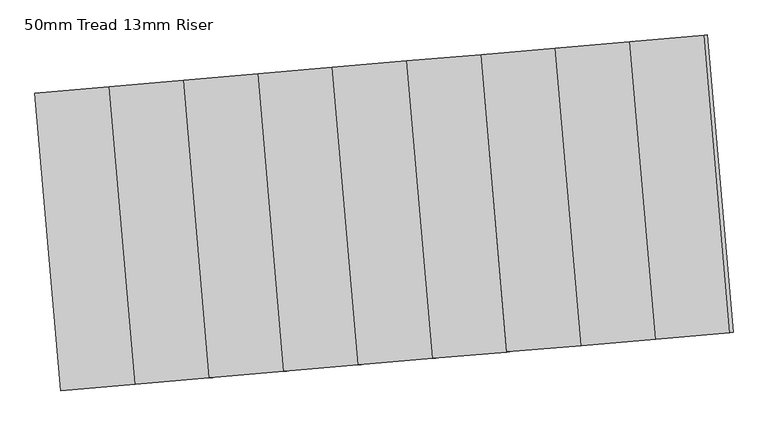
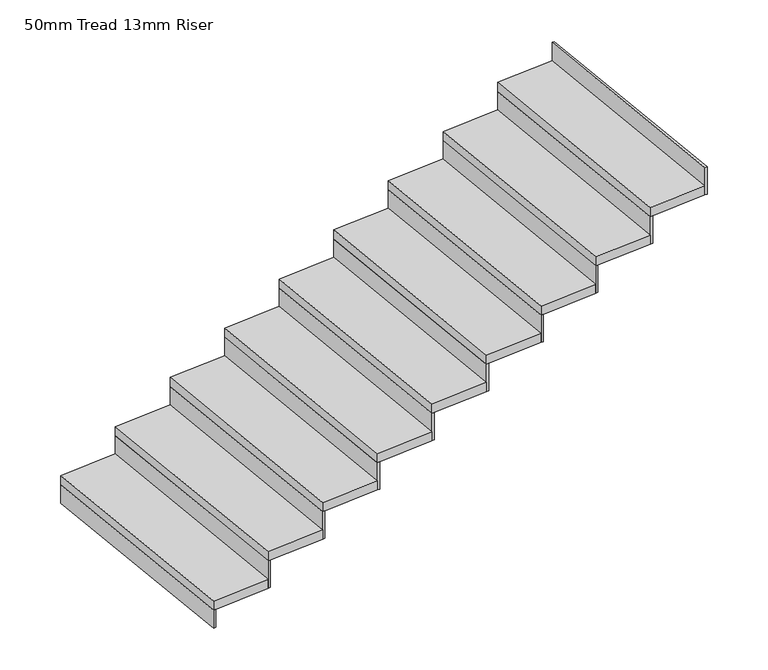
"""IFC4 building model written with IfcOpenShell, lengths in millimetres: stair flight geometry, 50mm Tread 13mm Riser."""

from ifc_helpers import new_model, si_unit, frame, origin, origin_with_axes, place, context, project, spatial, polyline, outline, extrude, source, transform, mapped, element, save


def stair_flight_50mm_tread_13mm_riser_4faf30c2(model_context):
    return source(origin(), model_context, "Body", "SweptSolid", [
        extrude(outline(polyline([(-18807.6730191, 13282.2135061), (-18820.126331, 13281.1341437), (-18923.7451249, 14476.652084), (-18911.2918131, 14477.7314464), (-18807.6730191, 13282.2135061)])), origin_with_axes(), (0.0, 0.0, 1.0), 100.0),
        extrude(outline(polyline([(-18624.8656399, 14502.5567824), (-18521.2468459, 13307.0388422), (-18820.126331, 13281.1341437), (-18923.7451249, 14476.652084), (-18624.8656399, 14502.5567824)])), frame((0.0, 0.0, 100.0), z_axis=(0.0, 0.0, 1.0), x_axis=(1.0, 0.0, 0.0)), (0.0, 0.0, 1.0), 50.0),
        extrude(outline(polyline([(-18508.793534, 13308.1182046), (-18521.2468459, 13307.0388422), (-18624.8656399, 14502.5567824), (-18612.412328, 14503.6361449), (-18508.793534, 13308.1182046)])), frame((0.0, 0.0, 100.0), z_axis=(0.0, 0.0, 1.0), x_axis=(1.0, 0.0, 0.0)), (0.0, 0.0, 1.0), 150.0),
        extrude(outline(polyline([(-18325.9861548, 14528.4614809), (-18222.3673608, 13332.9435406), (-18521.2468459, 13307.0388422), (-18624.8656399, 14502.5567824), (-18325.9861548, 14528.4614809)])), frame((0.0, 0.0, 250.0), z_axis=(0.0, 0.0, 1.0), x_axis=(1.0, 0.0, 0.0)), (0.0, 0.0, 1.0), 50.0),
        extrude(outline(polyline([(-18209.914049, 13334.0229031), (-18222.3673608, 13332.9435406), (-18325.9861548, 14528.4614809), (-18313.5328429, 14529.5408434), (-18209.914049, 13334.0229031)])), frame((0.0, 0.0, 250.0), z_axis=(0.0, 0.0, 1.0), x_axis=(1.0, 0.0, 0.0)), (0.0, 0.0, 1.0), 150.0),
        extrude(outline(polyline([(-18027.1066697, 14554.3661794), (-17923.4878758, 13358.8482391), (-18222.3673608, 13332.9435406), (-18325.9861548, 14528.4614809), (-18027.1066697, 14554.3661794)])), frame((0.0, 0.0, 400.0), z_axis=(0.0, 0.0, 1.0), x_axis=(1.0, 0.0, 0.0)), (0.0, 0.0, 1.0), 50.0),
        extrude(outline(polyline([(-17911.0345639, 13359.9276016), (-17923.4878758, 13358.8482391), (-18027.1066697, 14554.3661794), (-18014.6533578, 14555.4455419), (-17911.0345639, 13359.9276016)])), frame((0.0, 0.0, 400.0), z_axis=(0.0, 0.0, 1.0), x_axis=(1.0, 0.0, 0.0)), (0.0, 0.0, 1.0), 150.0),
        extrude(outline(polyline([(-17728.2271846, 14580.2708779), (-17624.6083907, 13384.7529376), (-17923.4878758, 13358.8482391), (-18027.1066697, 14554.3661794), (-17728.2271846, 14580.2708779)])), frame((0.0, 0.0, 550.0), z_axis=(0.0, 0.0, 1.0), x_axis=(1.0, 0.0, 0.0)), (0.0, 0.0, 1.0), 50.0),
        extrude(outline(polyline([(-17612.1550788, 13385.8323001), (-17624.6083907, 13384.7529376), (-17728.2271846, 14580.2708779), (-17715.7738728, 14581.3502403), (-17612.1550788, 13385.8323001)])), frame((0.0, 0.0, 550.0), z_axis=(0.0, 0.0, 1.0), x_axis=(1.0, 0.0, 0.0)), (0.0, 0.0, 1.0), 150.0),
        extrude(outline(polyline([(-17429.3476996, 14606.1755764), (-17325.7289056, 13410.6576361), (-17624.6083907, 13384.7529376), (-17728.2271846, 14580.2708779), (-17429.3476996, 14606.1755764)])), frame((0.0, 0.0, 700.0), z_axis=(0.0, 0.0, 1.0), x_axis=(1.0, 0.0, 0.0)), (0.0, 0.0, 1.0), 50.0),
        extrude(outline(polyline([(-17313.2755937, 13411.7369985), (-17325.7289056, 13410.6576361), (-17429.3476996, 14606.1755764), (-17416.8943877, 14607.2549388), (-17313.2755937, 13411.7369985)])), frame((0.0, 0.0, 700.0), z_axis=(0.0, 0.0, 1.0), x_axis=(1.0, 0.0, 0.0)), (0.0, 0.0, 1.0), 150.0),
        extrude(outline(polyline([(-17130.4682145, 14632.0802749), (-17026.8494206, 13436.5623346), (-17325.7289056, 13410.6576361), (-17429.3476996, 14606.1755764), (-17130.4682145, 14632.0802749)])), frame((0.0, 0.0, 850.0), z_axis=(0.0, 0.0, 1.0), x_axis=(1.0, 0.0, 0.0)), (0.0, 0.0, 1.0), 50.0),
        extrude(outline(polyline([(-17014.3961087, 13437.641697), (-17026.8494206, 13436.5623346), (-17130.4682145, 14632.0802749), (-17118.0149026, 14633.1596373), (-17014.3961087, 13437.641697)])), frame((0.0, 0.0, 850.0), z_axis=(0.0, 0.0, 1.0), x_axis=(1.0, 0.0, 0.0)), (0.0, 0.0, 1.0), 150.0),
        extrude(outline(polyline([(-16831.5887294, 14657.9849734), (-16727.9699355, 13462.4670331), (-17026.8494206, 13436.5623346), (-17130.4682145, 14632.0802749), (-16831.5887294, 14657.9849734)])), frame((0.0, 0.0, 1000.0), z_axis=(0.0, 0.0, 1.0), x_axis=(1.0, 0.0, 0.0)), (0.0, 0.0, 1.0), 50.0),
        extrude(outline(polyline([(-16715.5166236, 13463.5463955), (-16727.9699355, 13462.4670331), (-16831.5887294, 14657.9849734), (-16819.1354176, 14659.0643358), (-16715.5166236, 13463.5463955)])), frame((0.0, 0.0, 1000.0), z_axis=(0.0, 0.0, 1.0), x_axis=(1.0, 0.0, 0.0)), (0.0, 0.0, 1.0), 150.0),
        extrude(outline(polyline([(-16532.7092444, 14683.8896719), (-16429.0904504, 13488.3717316), (-16727.9699355, 13462.4670331), (-16831.5887294, 14657.9849734), (-16532.7092444, 14683.8896719)])), frame((0.0, 0.0, 1150.0), z_axis=(0.0, 0.0, 1.0), x_axis=(1.0, 0.0, 0.0)), (0.0, 0.0, 1.0), 50.0),
        extrude(outline(polyline([(-16416.6371385, 13489.451094), (-16429.0904504, 13488.3717316), (-16532.7092444, 14683.8896719), (-16520.2559325, 14684.9690343), (-16416.6371385, 13489.451094)])), frame((0.0, 0.0, 1150.0), z_axis=(0.0, 0.0, 1.0), x_axis=(1.0, 0.0, 0.0)), (0.0, 0.0, 1.0), 150.0),
        extrude(outline(polyline([(-16117.7576535, 13515.3557925), (-16130.2109653, 13514.2764301), (-16233.8297593, 14709.7943703), (-16221.3764474, 14710.8737328), (-16117.7576535, 13515.3557925)])), frame((0.0, 0.0, 1300.0), z_axis=(0.0, 0.0, 1.0), x_axis=(1.0, 0.0, 0.0)), (0.0, 0.0, 1.0), 150.0),
        extrude(outline(polyline([(-16233.8297593, 14709.7943703), (-16130.2109653, 13514.2764301), (-16429.0904504, 13488.3717316), (-16532.7092444, 14683.8896719), (-16233.8297593, 14709.7943703)])), frame((0.0, 0.0, 1300.0), z_axis=(0.0, 0.0, 1.0), x_axis=(1.0, 0.0, 0.0)), (0.0, 0.0, 1.0), 50.0),
    ])


if __name__ == "__main__":
    model = new_model("IFC4")
    model_context = context("Model", 3, world=origin())
    ifc_project = project(units=[si_unit("LENGTHUNIT", "METRE", prefix="MILLI")], contexts=[model_context])
    site = spatial("IfcSite", under=ifc_project)
    building = spatial("IfcBuilding", under=site)
    placement = place(None, origin())
    stair_flight_50mm_tread_13mm_riser_shape = stair_flight_50mm_tread_13mm_riser_4faf30c2(model_context)
    element("IfcStairFlight", 1, ObjectType="50mm Tread 13mm Riser", at=placement, inside=building, context=model_context, shape_type="MappedRepresentation", body=[
        mapped(stair_flight_50mm_tread_13mm_riser_shape, transform((0.0, 0.0, 0.0), x_axis=(1.0, 0.0, 0.0), y_axis=(0.0, 1.0, 0.0), z_axis=(0.0, 0.0, 1.0))),
    ])
    save(model, "model.ifc")

# Revit data of these elements
# Project information
#   Project Issue Date = "Issue Date"
#   Project Status = "Project Status"
#   Client Name = "Owner"
#   Project Address = "Enter address here"
#   Project Name = "Project Name"
#   Project Number = "0001"
